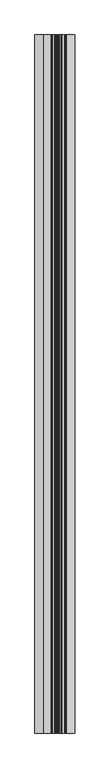
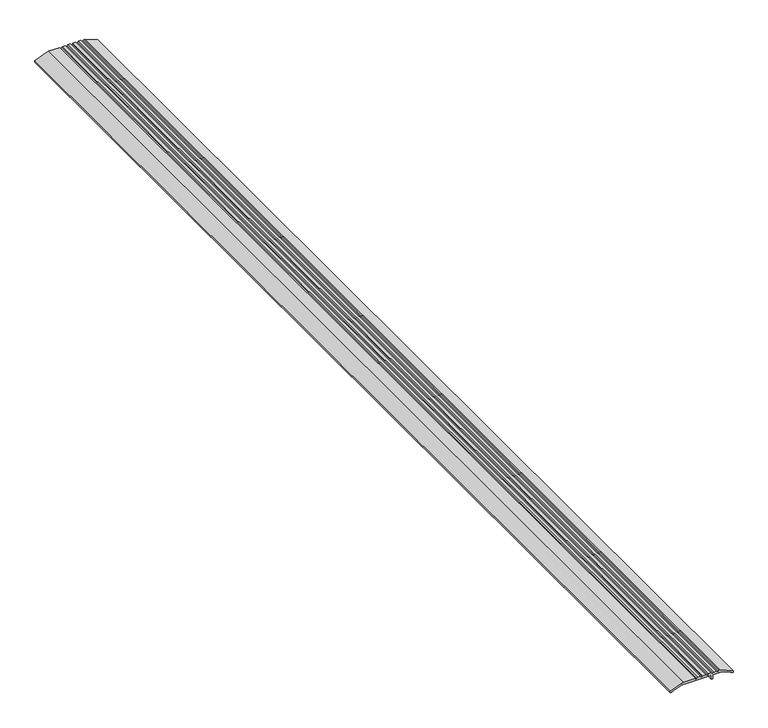
"""IFC4 building model written with IfcOpenShell, lengths in millimetres: proxy geometry, Door frame9:Door frame009:296264 : Door frame9:Door frame009:296264."""

from ifc_helpers import new_model, si_unit, frame, origin, place, context, project, spatial, polyline, outline, extrude, source, transform, mapped, element, save


def generic_models_5aac5b72(model_context):
    return source(origin(), model_context, "Body", "SweptSolid", [
        extrude(outline(polyline([(36580.0353123, 20347.4468857), (36582.0975353, 20346.2562607), (36582.0975353, 20341.3667607), (36580.0353123, 20340.1761357), (36580.0353123, 20337.7948857), (36582.0975353, 20336.6042607), (36582.0975353, 20331.7147607), (36580.0353123, 20330.5241357), (36580.0353123, 20328.1428857), (36582.0975353, 20326.9522607), (36582.0975353, 20305.6995587), (36572.5243303, 20281.8355107), (36569.3983841, 20281.8355107), (36569.3983841, 20285.0105107), (36570.3770561, 20285.0105107), (36577.3350353, 20302.3553342), (36577.3350353, 20356.7640675), (36569.5937593, 20356.7640675), (36569.5937593, 20359.3069538), (36577.3350353, 20359.3069538), (36577.3350353, 20375.6156872), (36570.3770561, 20392.9605107), (36569.3983841, 20392.9605107), (36569.3983841, 20396.1355107), (36572.5243303, 20396.1355107), (36582.0975353, 20372.2714626), (36582.0975353, 20370.3227607), (36580.0353123, 20369.1321357), (36580.0353123, 20366.7508857), (36582.0975353, 20365.5602607), (36582.0975353, 20360.6707607), (36580.0353123, 20359.4801357), (36580.0353123, 20357.0988857), (36582.0975353, 20355.9082607), (36582.0975353, 20351.0187607), (36580.0353123, 20349.8281357), (36580.0353123, 20347.4468857)])), frame((0.0, -774.5581156, 0.0), z_axis=(0.0, 1.0, 0.0), x_axis=(0.0, 0.0, 1.0)), (0.0, 0.0, 1.0), 1999.85),
    ])


if __name__ == "__main__":
    model = new_model("IFC4")
    model_context = context("Model", 3, world=origin())
    ifc_project = project(units=[si_unit("LENGTHUNIT", "METRE", prefix="MILLI")], contexts=[model_context])
    site = spatial("IfcSite", under=ifc_project)
    building = spatial("IfcBuilding", under=site)
    placement = place(None, origin())
    generic_models_shape = generic_models_5aac5b72(model_context)
    element("IfcBuildingElementProxy", 1, Name="Door frame9:Door frame009:296264 : Door frame9:Door frame009:296264", ObjectType="Door frame9:Door frame009:296264 : Door frame9:Door frame009:296264", at=placement, inside=building, context=model_context, shape_type="MappedRepresentation", body=[
        mapped(generic_models_shape, transform((0.0, 0.0, 0.0), x_axis=(1.0, 0.0, 0.0), y_axis=(0.0, 1.0, 0.0), z_axis=(0.0, 0.0, 1.0))),
    ])
    save(model, "model.ifc")

# Revit data of these elements
# Type "Door frame9:Door frame009:296264 : Door frame9:Door frame009:296264"
#   NameOverride = "Door frame9:Door frame009:296264"
#   ObjectTypeOverride = "Door frame9:Door frame009"
#   Reference = "Door frame009"
#   Category = "Generic Models"
#   Tag = "296264"
# Element 1 (IfcBuildingElementProxy, "Door frame9:Door frame009:296264 : Door frame9:Door frame009:296264")
#   Materials on its faces: "ALUM. THRESHOLD 171171"
# Materials
#   "ALUM. THRESHOLD 171171": class "Unassigned", colour RGB 247 247 247, transparency 0
